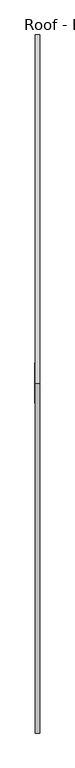
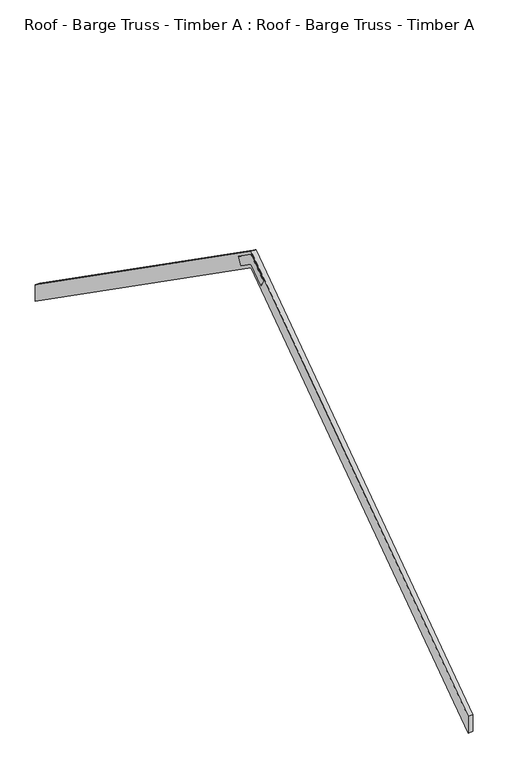
"""IFC4 building model written with IfcOpenShell, lengths in millimetres: furniture geometry, Roof - Barge Truss - Timber A : Roof - Barge Truss - Timber A."""

from ifc_helpers import new_model, si_unit, frame, origin, place, context, project, spatial, polyline, outline, extrude, source, transform, mapped, element, save


def roof_barge_truss_timber_a_roof_barge_truss_timber_a_2ed991f7(model_context):
    return source(origin(), model_context, "Body", "SweptSolid", [
        extrude(outline(polyline([(-300.0, 2810.9005033), (3620.25, 65.9119017), (3620.25, -117.2042867), (-300.0, 2627.784315), (-4239.4775971, -130.6675951), (-4239.4775971, 52.4485932), (-300.0, 2810.9005033)])), frame((19.8827307, 0.0, 0.0), z_axis=(1.0, 0.0, 0.0), x_axis=(0.0, 1.0, 0.0)), (0.0, 0.0, 1.0), 49.6351915),
        extrude(outline(polyline([(-299.7806483, 2778.8151222), (-72.8793639, 2619.9371325), (-119.3123526, 2542.6596622), (-299.7238694, 2668.9851662), (-480.2153155, 2542.6036951), (-526.6819326, 2619.9371325), (-299.7806483, 2778.8151222)])), frame((17.4104988, 0.0, 0.0), z_axis=(1.0, 0.0, 0.0), x_axis=(0.0, 1.0, 0.0)), (0.0, 0.0, 1.0), 2.4722319),
        extrude(outline(polyline([(-299.7806483, 2777.9554848), (-72.8793639, 2619.0774951), (-119.345981, 2541.7440577), (-299.7806483, 2668.0857719), (-480.2153155, 2541.7440577), (-526.6819326, 2619.0774951), (-299.7806483, 2777.9554848)])), frame((69.5179222, 0.0, 0.0), z_axis=(1.0, 0.0, 0.0), x_axis=(0.0, 1.0, 0.0)), (0.0, 0.0, 1.0), 2.0827493),
    ])


if __name__ == "__main__":
    model = new_model("IFC4")
    model_context = context("Model", 3, world=origin())
    ifc_project = project(units=[si_unit("LENGTHUNIT", "METRE", prefix="MILLI")], contexts=[model_context])
    site = spatial("IfcSite", under=ifc_project)
    building = spatial("IfcBuilding", under=site)
    placement = place(None, origin())
    roof_barge_truss_timber_a_roof_barge_truss_timber_a_shape = roof_barge_truss_timber_a_roof_barge_truss_timber_a_2ed991f7(model_context)
    element("IfcFurniture", 1, ObjectType="Roof - Barge Truss - Timber A : Roof - Barge Truss - Timber A", at=placement, inside=building, context=model_context, shape_type="MappedRepresentation", body=[
        mapped(roof_barge_truss_timber_a_roof_barge_truss_timber_a_shape, transform((0.0, 0.0, 0.0), x_axis=(1.0, 0.0, 0.0), y_axis=(0.0, 1.0, 0.0), z_axis=(0.0, 0.0, 1.0))),
    ])
    save(model, "model.ifc")

# Revit data of these elements
# Type "Roof - Barge Truss - Timber A : Roof - Barge Truss - Timber A"
#   Manufacturer = "M W Roofs"
#   Finish = "Rough"
#   Description = "Preformed Gangnail Barge ladder Truss"
#   Construction Type = "Timber"
#   Depth = 600 mm
#   Height = 900 mm
#   Width = 900 mm
# Element 1 (IfcFurniture, "Roof - Barge Truss - Timber A : Roof - Barge Truss - Timber A")
#   Materials on its faces: "Softwood, Lumber"
# Materials
#   "Softwood, Lumber": class "Wood", colour RGB 205 156 65, transparency 0, Description = "Pinus Echinata", Cost = 0
